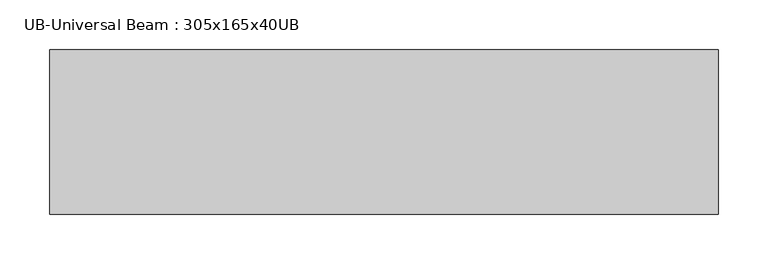
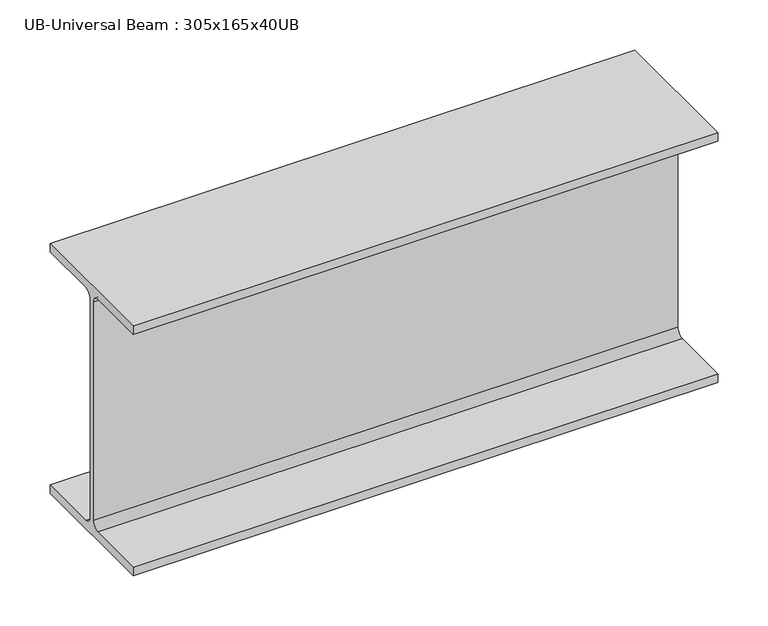
"""IFC4 building model written with IfcOpenShell, lengths in millimetres: beam geometry, UB-Universal Beam : 305x165x40UB."""

from ifc_helpers import new_model, si_unit, point, frame, frame_2d, origin, place, context, project, spatial, polyline, circle_curve, trimmed, segment, composite_curve, outline, extrude, source, transform, mapped, element, save


def ub_universal_beam_305x165x40ub_24de31be(model_context):
    return source(origin(), model_context, "Body", "SweptSolid", [
        extrude(outline(composite_curve([segment(polyline([(82.5, -141.5), (82.5, -151.7), (-82.5, -151.7), (-82.5, -141.5), (-11.9, -141.5)]), True, "CONTINUOUS"), segment(trimmed(circle_curve(frame_2d((-11.9, -132.6)), 8.9), [point((-11.9, -141.5))], [point((-3.0, -132.6))], True, "CARTESIAN"), True, "CONTINUOUS"), segment(polyline([(-3.0, -132.6), (-3.0, 132.6)]), True, "CONTINUOUS"), segment(trimmed(circle_curve(frame_2d((-11.9, 132.6)), 8.9), [point((-3.0, 132.6))], [point((-11.9, 141.5))], True, "CARTESIAN"), True, "CONTINUOUS"), segment(polyline([(-11.9, 141.5), (-82.5, 141.5), (-82.5, 151.7), (82.5, 151.7), (82.5, 141.5), (11.9, 141.5)]), True, "CONTINUOUS"), segment(trimmed(circle_curve(frame_2d((11.9, 132.6)), 8.9), [point((11.9, 141.5))], [point((3.0, 132.6))], True, "CARTESIAN"), True, "CONTINUOUS"), segment(polyline([(3.0, 132.6), (3.0, -132.6)]), True, "CONTINUOUS"), segment(trimmed(circle_curve(frame_2d((11.9, -132.6)), 8.9), [point((3.0, -132.6))], [point((11.9, -141.5))], True, "CARTESIAN"), True, "CONTINUOUS"), segment(polyline([(11.9, -141.5), (82.5, -141.5)]), True, "CONTINUOUS")], self_intersect=False)), frame((-335.6, 0.0, 0.0), z_axis=(1.0, 0.0, 0.0), x_axis=(0.0, 1.0, 0.0)), (0.0, 0.0, 1.0), 671.2),
    ])


if __name__ == "__main__":
    model = new_model("IFC4")
    model_context = context("Model", 3, world=origin())
    ifc_project = project(units=[si_unit("LENGTHUNIT", "METRE", prefix="MILLI")], contexts=[model_context])
    site = spatial("IfcSite", under=ifc_project)
    building = spatial("IfcBuilding", under=site)
    placement = place(None, origin())
    ub_universal_beam_305x165x40ub_shape = ub_universal_beam_305x165x40ub_24de31be(model_context)
    element("IfcBeam", 1, ObjectType="UB-Universal Beam : 305x165x40UB", at=placement, inside=building, context=model_context, shape_type="MappedRepresentation", body=[
        mapped(ub_universal_beam_305x165x40ub_shape, transform((0.0, 0.0, 0.0), x_axis=(1.0, 0.0, 0.0), y_axis=(0.0, 1.0, 0.0), z_axis=(0.0, 0.0, 1.0))),
    ])
    save(model, "model.ifc")

# Revit data of these elements
# Type "UB-Universal Beam : 305x165x40UB"
#   Nominal h = "305"
#   W = 0
#   Start Extension Calculation [instance default] = 3000 mm
#   Start Extension [instance default] = -12.7 mm
#   End Extension Calculation [instance default] = 3000 mm
#   End Extension [instance default] = -12.7 mm
#   Ix = 8503
#   Length [instance default] = 1524 mm
#   M = 40.3
#   Zx = 560
#   b = 165 mm
#   h = 303.4 mm
#   r = 8.9 mm
#   s = 6 mm
#   t = 10.2 mm
#   A = 0.005 m²
#   Structural Material [instance default] = Metal - Steel - 345 MPa
#   Assembly Code = ""
# Element 1 (IfcBeam, "UB-Universal Beam : 305x165x40UB")
#   Materials on its faces: "Metal - Steel - 345 MPa"
# Materials
#   "Metal - Steel - 345 MPa": class "Metal", colour RGB 241 46 46, transparency 0
